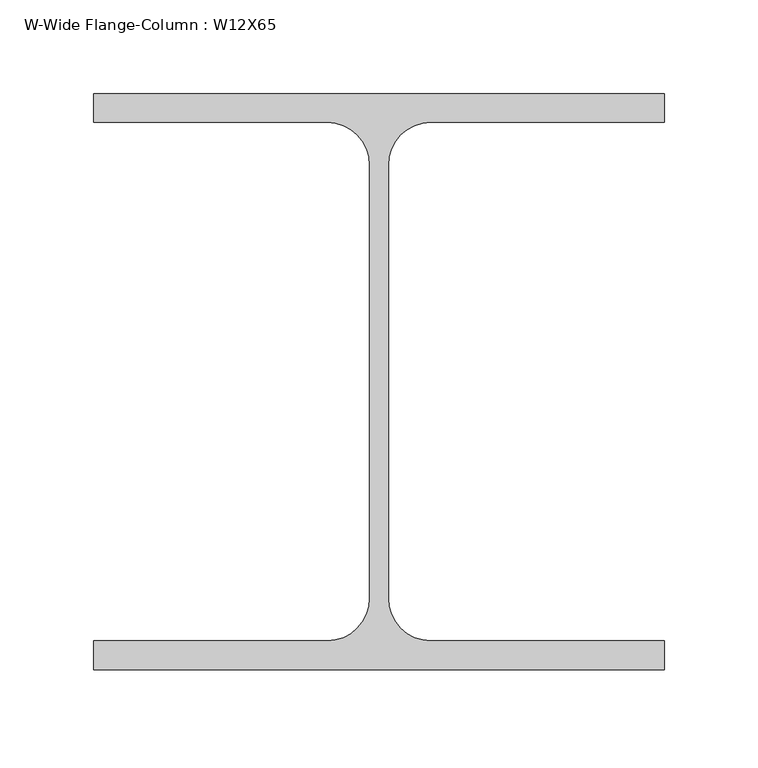
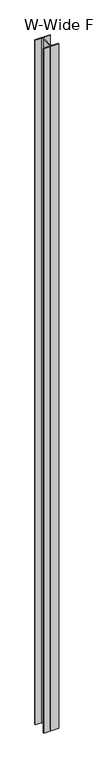
"""IFC4 building model written with IfcOpenShell, lengths in millimetres: column geometry, W-Wide Flange-Column : W12X65."""

import ifcopenshell
import ifcopenshell.guid

model = None  # the IFC model being written
_history = None  # IfcOwnerHistory: only IFC2X3 demands one
_inside = {}  # id of a spatial element -> (the spatial element, [elements in it])
_under = {}  # id of a project, library or spatial element -> (it, [spatial elements below it])
_declared = {}  # id of a project -> (the project, [libraries it declares])
_typed = {}  # id of a type object -> (the type object, [elements of that type])
_made_of = {}  # id of a material, layer set ... -> (it, [elements and type objects made of it])


def new_model(schema):
    """Start an empty IFC model of exactly this schema.

    Asked for "IFC4X3", IfcOpenShell would pick the latest addendum, in which some entities
    have other attributes; the version numbers below select the first issue.
    IFC2X3 requires an IfcOwnerHistory on every rooted entity: one is made here for all.
    """
    global model, _history
    if schema == "IFC4X3":
        model = ifcopenshell.file(schema_version=(4, 3, 0, 0))
    else:
        model = ifcopenshell.file(schema=schema)
    _inside.clear()
    _under.clear()
    _declared.clear()
    _typed.clear()
    _made_of.clear()
    _history = None
    if model.schema == "IFC2X3":
        org = make("IfcOrganization", Name="unknown")
        user = make(
            "IfcPersonAndOrganization",
            ThePerson=make("IfcPerson", FamilyName="unknown"),
            TheOrganization=org,
        )
        app = make(
            "IfcApplication",
            ApplicationDeveloper=org,
            Version="unknown",
            ApplicationFullName="unknown",
            ApplicationIdentifier="unknown",
        )
        _history = make(
            "IfcOwnerHistory",
            OwningUser=user,
            OwningApplication=app,
            ChangeAction="ADDED",
            CreationDate=0,
        )
    return model


def make(cls, **values):
    """One entity of the class cls with the attributes given. An attribute that is None is left unset."""
    return model.create_entity(
        cls, **{name: value for name, value in values.items() if value is not None}
    )


def rooted(cls, **values):
    """An entity with a GlobalId (a new one), such as an element, a storey or a relation."""
    return make(cls, GlobalId=ifcopenshell.guid.new(), OwnerHistory=_history, **values)


def si_unit(unit_type, name, prefix=None):
    """IfcSIUnit, for example si_unit("LENGTHUNIT", "METRE", prefix="MILLI")."""
    return make("IfcSIUnit", UnitType=unit_type, Prefix=prefix, Name=name)


def assignment(units):
    """IfcUnitAssignment: the units of a project."""
    return None if units is None else make("IfcUnitAssignment", Units=units)


def point(xyz):
    """IfcCartesianPoint."""
    return None if xyz is None else make("IfcCartesianPoint", Coordinates=xyz)


def direction(xyz):
    """IfcDirection."""
    return None if xyz is None else make("IfcDirection", DirectionRatios=xyz)


def frame(location, z_axis=None, x_axis=None):
    """IfcAxis2Placement3D, a coordinate frame: its origin and axes. An axis left out is left unset."""
    return make(
        "IfcAxis2Placement3D",
        Location=point(location),
        Axis=direction(z_axis),
        RefDirection=direction(x_axis),
    )


def frame_2d(location, x_axis=None):
    """IfcAxis2Placement2D, a coordinate frame in the plane: its origin and x axis."""
    return make(
        "IfcAxis2Placement2D", Location=point(location), RefDirection=direction(x_axis)
    )


def origin():
    """The frame at (0, 0, 0) with its axes left unset."""
    return frame((0.0, 0.0, 0.0))


def place(relative_to, where):
    """IfcLocalPlacement: puts the frame where relative to a parent placement (None: the world)."""
    return make(
        "IfcLocalPlacement", PlacementRelTo=relative_to, RelativePlacement=where
    )


def context(
    kind, dimensions, precision=None, world=None, true_north=None, identifier=None
):
    """IfcGeometricRepresentationContext, for example the 3D "Model" context."""
    return make(
        "IfcGeometricRepresentationContext",
        ContextIdentifier=identifier,
        ContextType=kind,
        CoordinateSpaceDimension=dimensions,
        Precision=precision,
        WorldCoordinateSystem=world,
        TrueNorth=true_north,
    )


def project(units=None, contexts=None):
    """IfcProject with its units and contexts."""
    return rooted(
        "IfcProject",
        Name="project",
        RepresentationContexts=contexts,
        UnitsInContext=assignment(units),
    )


def spatial(cls, under=None, at=None, **own):
    """A site, building, storey or space (cls), placed at a placement, below another one or the project."""
    s = rooted(cls, ObjectPlacement=at, **own)
    if under is not None:
        _under.setdefault(under.id(), (under, []))[1].append(s)
    return s


def polyline(points):
    """IfcPolyline through the points."""
    return make("IfcPolyline", Points=[point(p) for p in points])


def circle_curve(where, radius):
    """IfcCircle in the frame where."""
    return make("IfcCircle", Position=where, Radius=radius)


def trimmed(basis, trim1, trim2, sense, master):
    """IfcTrimmedCurve: the piece of a basis curve between two trims."""
    return make(
        "IfcTrimmedCurve",
        BasisCurve=basis,
        Trim1=trim1,
        Trim2=trim2,
        SenseAgreement=sense,
        MasterRepresentation=master,
    )


def segment(curve, same_sense, transition):
    """IfcCompositeCurveSegment."""
    return make(
        "IfcCompositeCurveSegment",
        Transition=transition,
        SameSense=same_sense,
        ParentCurve=curve,
    )


def composite_curve(segments, self_intersect=None):
    """IfcCompositeCurve: segments joined end to end."""
    return make("IfcCompositeCurve", Segments=segments, SelfIntersect=self_intersect)


def outline(outer, holes=None, kind="AREA"):
    """IfcArbitraryClosedProfileDef: a profile drawn as a closed curve; with holes, ...WithVoids."""
    if holes is None:
        return make("IfcArbitraryClosedProfileDef", ProfileType=kind, OuterCurve=outer)
    return make(
        "IfcArbitraryProfileDefWithVoids",
        ProfileType=kind,
        OuterCurve=outer,
        InnerCurves=holes,
    )


def extrude(swept, where, along, depth):
    """IfcExtrudedAreaSolid: the profile swept, set in the frame where, extruded along a direction by depth."""
    return make(
        "IfcExtrudedAreaSolid",
        SweptArea=swept,
        Position=where,
        ExtrudedDirection=direction(along),
        Depth=depth,
    )


def shape(context_of_items, identifier, shape_type, items):
    """IfcShapeRepresentation: the items that make up one representation, for example the "Body"."""
    return make(
        "IfcShapeRepresentation",
        ContextOfItems=context_of_items,
        RepresentationIdentifier=identifier,
        RepresentationType=shape_type,
        Items=items,
    )


def source(mapping_origin, context_of_items, identifier, shape_type, items):
    """IfcRepresentationMap: a shape defined once, which mapped items show again and again."""
    return make(
        "IfcRepresentationMap",
        MappingOrigin=mapping_origin,
        MappedRepresentation=shape(context_of_items, identifier, shape_type, items),
    )


def transform(
    local_origin,
    x_axis=None,
    y_axis=None,
    z_axis=None,
    scale=None,
    scale2=None,
    scale3=None,
    uniform=True,
):
    """IfcCartesianTransformationOperator3D, or its non-uniform kind. x_axis, y_axis, z_axis: its Axis1, 2, 3."""
    if uniform:
        return make(
            "IfcCartesianTransformationOperator3D",
            Axis1=direction(x_axis),
            Axis2=direction(y_axis),
            LocalOrigin=point(local_origin),
            Scale=scale,
            Axis3=direction(z_axis),
        )
    return make(
        "IfcCartesianTransformationOperator3DnonUniform",
        Axis1=direction(x_axis),
        Axis2=direction(y_axis),
        LocalOrigin=point(local_origin),
        Scale=scale,
        Axis3=direction(z_axis),
        Scale2=scale2,
        Scale3=scale3,
    )


def mapped(mapping_source, mapping_target):
    """IfcMappedItem: shows the shape of a source again, moved by a transform."""
    return make(
        "IfcMappedItem", MappingSource=mapping_source, MappingTarget=mapping_target
    )


def made_of(thing, what):
    """Note that an element or type object is made of a material, layer set ...; save() writes the relation."""
    if what is not None:
        _made_of.setdefault(what.id(), (what, []))[1].append(thing)
    return thing


def element(
    cls,
    number,
    at=None,
    inside=None,
    cuts=None,
    type_object=None,
    material=None,
    context=None,
    identifier="Body",
    shape_type=None,
    held_by="IfcProductDefinitionShape",
    body=None,
    shapes=None,
    **own,
):
    """One element of the class cls, such as IfcWall. Its Tag is "e" and its number.

    at: its placement. inside: the storey or other place that contains it. cuts: it is an
    opening in that element (IfcRelVoidsElement). A single representation is given by context,
    identifier, shape_type and body (its items); several are given by shapes. held_by: the class
    of the entity that holds the representations. save() writes the other relations.
    """
    e = rooted(cls, Tag="e%d" % number, ObjectPlacement=at, **own)
    if body is not None:
        shapes = [shape(context, identifier, shape_type, body)]
    if shapes is not None:
        e.Representation = make(held_by, Representations=shapes)
    if inside is not None:
        _inside.setdefault(inside.id(), (inside, []))[1].append(e)
    if cuts is not None:
        rooted(
            "IfcRelVoidsElement", RelatingBuildingElement=cuts, RelatedOpeningElement=e
        )
    if type_object is not None:
        _typed.setdefault(type_object.id(), (type_object, []))[1].append(e)
    return made_of(e, material)


def aggregate(whole, parts):
    """IfcRelAggregates: a whole, such as a stair, and the parts it consists of."""
    return rooted("IfcRelAggregates", RelatingObject=whole, RelatedObjects=parts)


def save(model, path):
    """Write the relations noted so far, then the file.

    IfcRelAggregates (storeys below a building ...), IfcRelContainedInSpatialStructure (elements
    in a storey), IfcRelDefinesByType, IfcRelAssociatesMaterial and IfcRelDeclares: one each for
    every whole, place, type object, material and project.
    """
    for whole, parts in _under.values():
        aggregate(whole, parts)
    for where, things in _inside.values():
        rooted(
            "IfcRelContainedInSpatialStructure",
            RelatedElements=things,
            RelatingStructure=where,
        )
    for kind, things in _typed.values():
        rooted("IfcRelDefinesByType", RelatedObjects=things, RelatingType=kind)
    for what, things in _made_of.values():
        rooted("IfcRelAssociatesMaterial", RelatedObjects=things, RelatingMaterial=what)
    for by, libraries in _declared.values():
        rooted("IfcRelDeclares", RelatingContext=by, RelatedDefinitions=libraries)
    model.write(path)


def w_wide_flange_column_w12x65_b7a4a025(model_context):
    return source(origin(), model_context, "Body", "SweptSolid", [
        extrude(outline(composite_curve([segment(polyline([(152.4, 153.67), (152.4, 138.303), (27.686, 138.303)]), True, "CONTINUOUS"), segment(trimmed(circle_curve(frame_2d((27.686, 115.57)), 22.733), [point((27.686, 138.303))], [point((4.953, 115.57))], True, "CARTESIAN"), True, "CONTINUOUS"), segment(polyline([(4.953, 115.57), (4.953, -115.57)]), True, "CONTINUOUS"), segment(trimmed(circle_curve(frame_2d((27.686, -115.57)), 22.733), [point((4.953, -115.57))], [point((27.686, -138.303))], True, "CARTESIAN"), True, "CONTINUOUS"), segment(polyline([(27.686, -138.303), (152.4, -138.303), (152.4, -153.67), (-152.4, -153.67), (-152.4, -138.303), (-27.686, -138.303)]), True, "CONTINUOUS"), segment(trimmed(circle_curve(frame_2d((-27.686, -115.57)), 22.733), [point((-27.686, -138.303))], [point((-4.953, -115.57))], True, "CARTESIAN"), True, "CONTINUOUS"), segment(polyline([(-4.953, -115.57), (-4.953, 115.57)]), True, "CONTINUOUS"), segment(trimmed(circle_curve(frame_2d((-27.686, 115.57)), 22.733), [point((-4.953, 115.57))], [point((-27.686, 138.303))], True, "CARTESIAN"), True, "CONTINUOUS"), segment(polyline([(-27.686, 138.303), (-152.4, 138.303), (-152.4, 153.67), (152.4, 153.67)]), True, "CONTINUOUS")], self_intersect=False)), frame((0.0, 0.0, 8756.65), z_axis=(0.0, 0.0, 1.0), x_axis=(1.0, 0.0, 0.0)), (0.0, 0.0, 1.0), 14560.55),
    ])


if __name__ == "__main__":
    model = new_model("IFC4")
    model_context = context("Model", 3, world=origin())
    ifc_project = project(units=[si_unit("LENGTHUNIT", "METRE", prefix="MILLI")], contexts=[model_context])
    site = spatial("IfcSite", under=ifc_project)
    building = spatial("IfcBuilding", under=site)
    placement = place(None, origin())
    w_wide_flange_column_w12x65_shape = w_wide_flange_column_w12x65_b7a4a025(model_context)
    element("IfcColumn", 1, ObjectType="W-Wide Flange-Column : W12X65", at=placement, inside=building, context=model_context, shape_type="MappedRepresentation", body=[
        mapped(w_wide_flange_column_w12x65_shape, transform((0.0, 0.0, 0.0), x_axis=(1.0, 0.0, 0.0), y_axis=(0.0, 1.0, 0.0), z_axis=(0.0, 0.0, 1.0))),
    ])
    save(model, "model.ifc")

# Revit data of these elements
# Type "W-Wide Flange-Column : W12X65"
#   Assembly Code = "B10"
#   W = 65
#   bf = 1' - 0"
#   d = 1' - 0.1"
#   k = 0' - 1 1/2"
#   kr = 0' - 0.895"
#   tf = 0' - 0.605"
#   tw = 0' - 0.39"
#   A = 0.132639 SF
#   Structural Material [instance default] = Steel ASTM A992
# Element 1 (IfcColumn, "W-Wide Flange-Column : W12X65")
#   Materials on its faces: "Steel ASTM A992"
# Materials
#   "Steel ASTM A992": class "Metal", colour RGB 199 199 199, transparency 0, Description = "Structural steel 50ksi", Cost = 0
